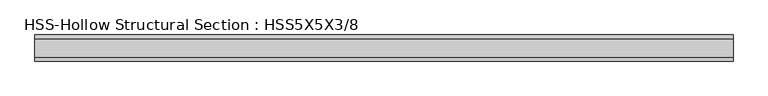
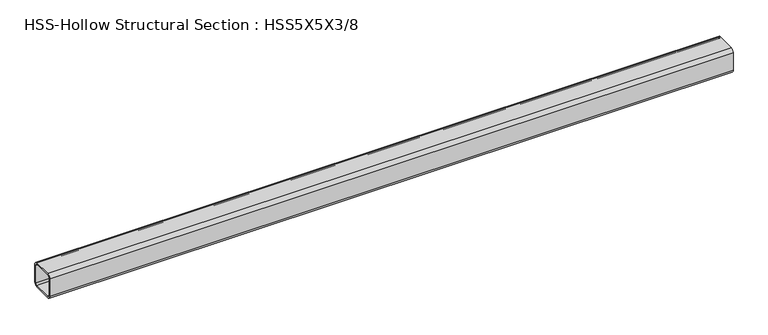
"""IFC4 building model written with IfcOpenShell, lengths in millimetres: member geometry, HSS-Hollow Structural Section : HSS5X5X3/8."""

from ifc_helpers import new_model, si_unit, point, frame, frame_2d, origin, place, context, project, spatial, polyline, circle_curve, trimmed, segment, composite_curve, outline, extrude, source, transform, mapped, element, save


def hss_hollow_structural_section_hss5x5x3_8_6dea9a89(model_context):
    return source(origin(), model_context, "Body", "SweptSolid", [
        extrude(outline(composite_curve([segment(polyline([(63.5, 45.7708), (63.5, -45.7708)]), True, "CONTINUOUS"), segment(trimmed(circle_curve(frame_2d((45.7708, -45.7708)), 17.7292), [point((63.5, -45.7708))], [point((45.7708, -63.5))], False, "CARTESIAN"), True, "CONTINUOUS"), segment(polyline([(45.7708, -63.5), (-45.7708, -63.5)]), True, "CONTINUOUS"), segment(trimmed(circle_curve(frame_2d((-45.7708, -45.7708)), 17.7292), [point((-45.7708, -63.5))], [point((-63.5, -45.7708))], False, "CARTESIAN"), True, "CONTINUOUS"), segment(polyline([(-63.5, -45.7708), (-63.5, 45.7708)]), True, "CONTINUOUS"), segment(trimmed(circle_curve(frame_2d((-45.7708, 45.7708)), 17.7292), [point((-63.5, 45.7708))], [point((-45.7708, 63.5))], False, "CARTESIAN"), True, "CONTINUOUS"), segment(polyline([(-45.7708, 63.5), (45.7708, 63.5)]), True, "CONTINUOUS"), segment(trimmed(circle_curve(frame_2d((45.7708, 45.7708)), 17.7292), [point((45.7708, 63.5))], [point((63.5, 45.7708))], False, "CARTESIAN"), True, "CONTINUOUS")], self_intersect=False), holes=[composite_curve([segment(trimmed(circle_curve(frame_2d((-45.7708, 45.7708)), 8.8646), [point((-45.7708, 54.6354))], [point((-54.6354, 45.7708))], True, "CARTESIAN"), True, "CONTINUOUS"), segment(polyline([(-54.6354, 45.7708), (-54.6354, -45.7708)]), True, "CONTINUOUS"), segment(trimmed(circle_curve(frame_2d((-45.7708, -45.7708)), 8.8646), [point((-54.6354, -45.7708))], [point((-45.7708, -54.6354))], True, "CARTESIAN"), True, "CONTINUOUS"), segment(polyline([(-45.7708, -54.6354), (45.7708, -54.6354)]), True, "CONTINUOUS"), segment(trimmed(circle_curve(frame_2d((45.7708, -45.7708)), 8.8646), [point((45.7708, -54.6354))], [point((54.6354, -45.7708))], True, "CARTESIAN"), True, "CONTINUOUS"), segment(polyline([(54.6354, -45.7708), (54.6354, 45.7708)]), True, "CONTINUOUS"), segment(trimmed(circle_curve(frame_2d((45.7708, 45.7708)), 8.8646), [point((54.6354, 45.7708))], [point((45.7708, 54.6354))], True, "CARTESIAN"), True, "CONTINUOUS"), segment(polyline([(45.7708, 54.6354), (-45.7708, 54.6354)]), True, "CONTINUOUS")], self_intersect=False)]), frame((-1658.4224836, 0.0, 0.0), z_axis=(1.0, 0.0, 0.0), x_axis=(0.0, 1.0, 0.0)), (0.0, 0.0, 1.0), 3392.5854856),
    ])


if __name__ == "__main__":
    model = new_model("IFC4")
    model_context = context("Model", 3, world=origin())
    ifc_project = project(units=[si_unit("LENGTHUNIT", "METRE", prefix="MILLI")], contexts=[model_context])
    site = spatial("IfcSite", under=ifc_project)
    building = spatial("IfcBuilding", under=site)
    placement = place(None, origin())
    hss_hollow_structural_section_hss5x5x3_8_shape = hss_hollow_structural_section_hss5x5x3_8_6dea9a89(model_context)
    element("IfcMember", 1, ObjectType="HSS-Hollow Structural Section : HSS5X5X3/8", at=placement, inside=building, context=model_context, shape_type="MappedRepresentation", body=[
        mapped(hss_hollow_structural_section_hss5x5x3_8_shape, transform((0.0, 0.0, 0.0), x_axis=(1.0, 0.0, 0.0), y_axis=(0.0, 1.0, 0.0), z_axis=(0.0, 0.0, 1.0))),
    ])
    save(model, "model.ifc")

# Revit data of these elements
# Type "HSS-Hollow Structural Section : HSS5X5X3/8"
#   Assembly Code = "B10"
#   Shape = "Square"
#   W = 22.3
#   Ht = 0' - 5"
#   Length [instance default] = 5' - 0"
#   b = 0' - 5"
#   kr = 0' - 0.698"
#   t = 0' - 0.349"
#   A = 0.0429167 SF
#   Structural Material [instance default] = Steel ASTM A500, Grade B, Rectangular and Square
# Element 1 (IfcMember, "HSS-Hollow Structural Section : HSS5X5X3/8")
#   Materials on its faces: "Steel ASTM A500, Grade B, Rectangular and Square"
# Materials
#   "Steel ASTM A500, Grade B, Rectangular and Square": class "Metal", colour RGB 199 199 199, transparency 0, Description = "Carbon steel", Cost = 0
